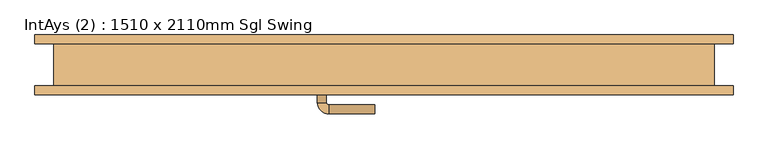
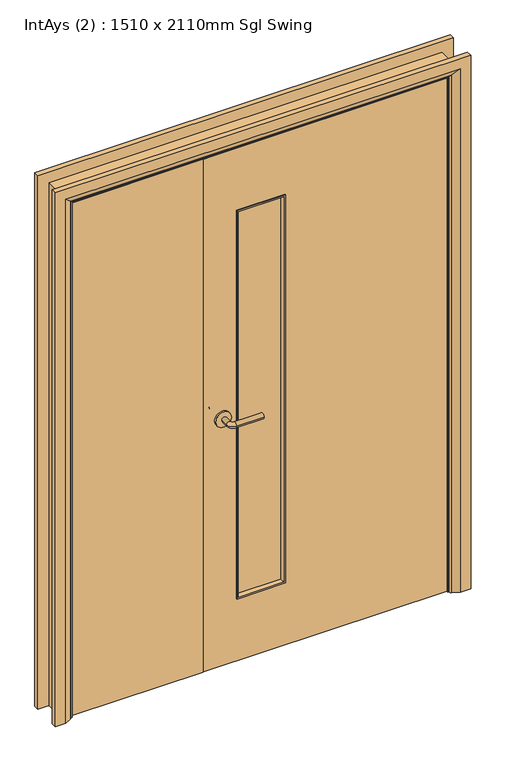
"""IFC4 building model written with IfcOpenShell, lengths in millimetres: door geometry, IntAys (2) : 1510 x 2110mm Sgl Swing."""

import ifcopenshell
import ifcopenshell.guid

model = None  # the IFC model being written
_history = None  # IfcOwnerHistory: only IFC2X3 demands one
_inside = {}  # id of a spatial element -> (the spatial element, [elements in it])
_under = {}  # id of a project, library or spatial element -> (it, [spatial elements below it])
_declared = {}  # id of a project -> (the project, [libraries it declares])
_typed = {}  # id of a type object -> (the type object, [elements of that type])
_made_of = {}  # id of a material, layer set ... -> (it, [elements and type objects made of it])


def new_model(schema):
    """Start an empty IFC model of exactly this schema.

    Asked for "IFC4X3", IfcOpenShell would pick the latest addendum, in which some entities
    have other attributes; the version numbers below select the first issue.
    IFC2X3 requires an IfcOwnerHistory on every rooted entity: one is made here for all.
    """
    global model, _history
    if schema == "IFC4X3":
        model = ifcopenshell.file(schema_version=(4, 3, 0, 0))
    else:
        model = ifcopenshell.file(schema=schema)
    _inside.clear()
    _under.clear()
    _declared.clear()
    _typed.clear()
    _made_of.clear()
    _history = None
    if model.schema == "IFC2X3":
        org = make("IfcOrganization", Name="unknown")
        user = make(
            "IfcPersonAndOrganization",
            ThePerson=make("IfcPerson", FamilyName="unknown"),
            TheOrganization=org,
        )
        app = make(
            "IfcApplication",
            ApplicationDeveloper=org,
            Version="unknown",
            ApplicationFullName="unknown",
            ApplicationIdentifier="unknown",
        )
        _history = make(
            "IfcOwnerHistory",
            OwningUser=user,
            OwningApplication=app,
            ChangeAction="ADDED",
            CreationDate=0,
        )
    return model


def make(cls, **values):
    """One entity of the class cls with the attributes given. An attribute that is None is left unset."""
    return model.create_entity(
        cls, **{name: value for name, value in values.items() if value is not None}
    )


def rooted(cls, **values):
    """An entity with a GlobalId (a new one), such as an element, a storey or a relation."""
    return make(cls, GlobalId=ifcopenshell.guid.new(), OwnerHistory=_history, **values)


def si_unit(unit_type, name, prefix=None):
    """IfcSIUnit, for example si_unit("LENGTHUNIT", "METRE", prefix="MILLI")."""
    return make("IfcSIUnit", UnitType=unit_type, Prefix=prefix, Name=name)


def assignment(units):
    """IfcUnitAssignment: the units of a project."""
    return None if units is None else make("IfcUnitAssignment", Units=units)


def point(xyz):
    """IfcCartesianPoint."""
    return None if xyz is None else make("IfcCartesianPoint", Coordinates=xyz)


def direction(xyz):
    """IfcDirection."""
    return None if xyz is None else make("IfcDirection", DirectionRatios=xyz)


def frame(location, z_axis=None, x_axis=None):
    """IfcAxis2Placement3D, a coordinate frame: its origin and axes. An axis left out is left unset."""
    return make(
        "IfcAxis2Placement3D",
        Location=point(location),
        Axis=direction(z_axis),
        RefDirection=direction(x_axis),
    )


def frame_2d(location, x_axis=None):
    """IfcAxis2Placement2D, a coordinate frame in the plane: its origin and x axis."""
    return make(
        "IfcAxis2Placement2D", Location=point(location), RefDirection=direction(x_axis)
    )


def origin():
    """The frame at (0, 0, 0) with its axes left unset."""
    return frame((0.0, 0.0, 0.0))


def place(relative_to, where):
    """IfcLocalPlacement: puts the frame where relative to a parent placement (None: the world)."""
    return make(
        "IfcLocalPlacement", PlacementRelTo=relative_to, RelativePlacement=where
    )


def context(
    kind, dimensions, precision=None, world=None, true_north=None, identifier=None
):
    """IfcGeometricRepresentationContext, for example the 3D "Model" context."""
    return make(
        "IfcGeometricRepresentationContext",
        ContextIdentifier=identifier,
        ContextType=kind,
        CoordinateSpaceDimension=dimensions,
        Precision=precision,
        WorldCoordinateSystem=world,
        TrueNorth=true_north,
    )


def project(units=None, contexts=None):
    """IfcProject with its units and contexts."""
    return rooted(
        "IfcProject",
        Name="project",
        RepresentationContexts=contexts,
        UnitsInContext=assignment(units),
    )


def spatial(cls, under=None, at=None, **own):
    """A site, building, storey or space (cls), placed at a placement, below another one or the project."""
    s = rooted(cls, ObjectPlacement=at, **own)
    if under is not None:
        _under.setdefault(under.id(), (under, []))[1].append(s)
    return s


def polyline(points):
    """IfcPolyline through the points."""
    return make("IfcPolyline", Points=[point(p) for p in points])


def circle_curve(where, radius):
    """IfcCircle in the frame where."""
    return make("IfcCircle", Position=where, Radius=radius)


def ellipse_curve(where, semi_axis1, semi_axis2):
    """IfcEllipse in the frame where."""
    return make(
        "IfcEllipse", Position=where, SemiAxis1=semi_axis1, SemiAxis2=semi_axis2
    )


def trimmed(basis, trim1, trim2, sense, master):
    """IfcTrimmedCurve: the piece of a basis curve between two trims."""
    return make(
        "IfcTrimmedCurve",
        BasisCurve=basis,
        Trim1=trim1,
        Trim2=trim2,
        SenseAgreement=sense,
        MasterRepresentation=master,
    )


def segment(curve, same_sense, transition):
    """IfcCompositeCurveSegment."""
    return make(
        "IfcCompositeCurveSegment",
        Transition=transition,
        SameSense=same_sense,
        ParentCurve=curve,
    )


def composite_curve(segments, self_intersect=None):
    """IfcCompositeCurve: segments joined end to end."""
    return make("IfcCompositeCurve", Segments=segments, SelfIntersect=self_intersect)


def outline(outer, holes=None, kind="AREA"):
    """IfcArbitraryClosedProfileDef: a profile drawn as a closed curve; with holes, ...WithVoids."""
    if holes is None:
        return make("IfcArbitraryClosedProfileDef", ProfileType=kind, OuterCurve=outer)
    return make(
        "IfcArbitraryProfileDefWithVoids",
        ProfileType=kind,
        OuterCurve=outer,
        InnerCurves=holes,
    )


def extrude(swept, where, along, depth):
    """IfcExtrudedAreaSolid: the profile swept, set in the frame where, extruded along a direction by depth."""
    return make(
        "IfcExtrudedAreaSolid",
        SweptArea=swept,
        Position=where,
        ExtrudedDirection=direction(along),
        Depth=depth,
    )


def faces_of(points, faces, orient=None, outer=None):
    """IfcFace entities. A face is a list of loops; a loop is a list of indices into points, from 0.

    orient and outer hold one flag for each loop. By default every Orientation is true, the
    first loop of a face is its IfcFaceOuterBound and the others are IfcFaceBound.
    """
    made = []
    for i, loops in enumerate(faces):
        bounds = []
        for j, loop in enumerate(loops):
            is_outer = j == 0 if outer is None else outer[i][j]
            bounds.append(
                make(
                    "IfcFaceOuterBound" if is_outer else "IfcFaceBound",
                    Bound=make("IfcPolyLoop", Polygon=[points[k] for k in loop]),
                    Orientation=True if orient is None else orient[i][j],
                )
            )
        made.append(make("IfcFace", Bounds=bounds))
    return made


def faceted_brep(points, faces, orient=None, outer=None, voids=None):
    """IfcFacetedBrep: a solid bounded by flat faces; with voids (closed shells), ...WithVoids."""
    shared = [point(p) for p in points]
    hull = make("IfcClosedShell", CfsFaces=faces_of(shared, faces, orient, outer))
    if voids is None:
        return make("IfcFacetedBrep", Outer=hull)
    return make(
        "IfcFacetedBrepWithVoids",
        Outer=hull,
        Voids=[
            make(cls, CfsFaces=faces_of(shared, fs, o, b)) for cls, fs, o, b in voids
        ],
    )


def shape(context_of_items, identifier, shape_type, items):
    """IfcShapeRepresentation: the items that make up one representation, for example the "Body"."""
    return make(
        "IfcShapeRepresentation",
        ContextOfItems=context_of_items,
        RepresentationIdentifier=identifier,
        RepresentationType=shape_type,
        Items=items,
    )


def source(mapping_origin, context_of_items, identifier, shape_type, items):
    """IfcRepresentationMap: a shape defined once, which mapped items show again and again."""
    return make(
        "IfcRepresentationMap",
        MappingOrigin=mapping_origin,
        MappedRepresentation=shape(context_of_items, identifier, shape_type, items),
    )


def transform(
    local_origin,
    x_axis=None,
    y_axis=None,
    z_axis=None,
    scale=None,
    scale2=None,
    scale3=None,
    uniform=True,
):
    """IfcCartesianTransformationOperator3D, or its non-uniform kind. x_axis, y_axis, z_axis: its Axis1, 2, 3."""
    if uniform:
        return make(
            "IfcCartesianTransformationOperator3D",
            Axis1=direction(x_axis),
            Axis2=direction(y_axis),
            LocalOrigin=point(local_origin),
            Scale=scale,
            Axis3=direction(z_axis),
        )
    return make(
        "IfcCartesianTransformationOperator3DnonUniform",
        Axis1=direction(x_axis),
        Axis2=direction(y_axis),
        LocalOrigin=point(local_origin),
        Scale=scale,
        Axis3=direction(z_axis),
        Scale2=scale2,
        Scale3=scale3,
    )


def mapped(mapping_source, mapping_target):
    """IfcMappedItem: shows the shape of a source again, moved by a transform."""
    return make(
        "IfcMappedItem", MappingSource=mapping_source, MappingTarget=mapping_target
    )


def made_of(thing, what):
    """Note that an element or type object is made of a material, layer set ...; save() writes the relation."""
    if what is not None:
        _made_of.setdefault(what.id(), (what, []))[1].append(thing)
    return thing


def element(
    cls,
    number,
    at=None,
    inside=None,
    cuts=None,
    type_object=None,
    material=None,
    context=None,
    identifier="Body",
    shape_type=None,
    held_by="IfcProductDefinitionShape",
    body=None,
    shapes=None,
    **own,
):
    """One element of the class cls, such as IfcWall. Its Tag is "e" and its number.

    at: its placement. inside: the storey or other place that contains it. cuts: it is an
    opening in that element (IfcRelVoidsElement). A single representation is given by context,
    identifier, shape_type and body (its items); several are given by shapes. held_by: the class
    of the entity that holds the representations. save() writes the other relations.
    """
    e = rooted(cls, Tag="e%d" % number, ObjectPlacement=at, **own)
    if body is not None:
        shapes = [shape(context, identifier, shape_type, body)]
    if shapes is not None:
        e.Representation = make(held_by, Representations=shapes)
    if inside is not None:
        _inside.setdefault(inside.id(), (inside, []))[1].append(e)
    if cuts is not None:
        rooted(
            "IfcRelVoidsElement", RelatingBuildingElement=cuts, RelatedOpeningElement=e
        )
    if type_object is not None:
        _typed.setdefault(type_object.id(), (type_object, []))[1].append(e)
    return made_of(e, material)


def aggregate(whole, parts):
    """IfcRelAggregates: a whole, such as a stair, and the parts it consists of."""
    return rooted("IfcRelAggregates", RelatingObject=whole, RelatedObjects=parts)


def save(model, path):
    """Write the relations noted so far, then the file.

    IfcRelAggregates (storeys below a building ...), IfcRelContainedInSpatialStructure (elements
    in a storey), IfcRelDefinesByType, IfcRelAssociatesMaterial and IfcRelDeclares: one each for
    every whole, place, type object, material and project.
    """
    for whole, parts in _under.values():
        aggregate(whole, parts)
    for where, things in _inside.values():
        rooted(
            "IfcRelContainedInSpatialStructure",
            RelatedElements=things,
            RelatingStructure=where,
        )
    for kind, things in _typed.values():
        rooted("IfcRelDefinesByType", RelatedObjects=things, RelatingType=kind)
    for what, things in _made_of.values():
        rooted("IfcRelAssociatesMaterial", RelatedObjects=things, RelatingMaterial=what)
    for by, libraries in _declared.values():
        rooted("IfcRelDeclares", RelatingContext=by, RelatedDefinitions=libraries)
    model.write(path)


def plane_surface(at):
    """IfcPlane: the flat surface through the origin of the frame at, square to its z axis."""
    return make("IfcPlane", Position=at)


def cylinder_surface(at, radius):
    """IfcCylindricalSurface: all points at the distance radius from the z axis of the frame at."""
    return make("IfcCylindricalSurface", Position=at, Radius=radius)


def revolved_surface(curve, axis_point, axis_direction):
    """IfcSurfaceOfRevolution: the curve turned about the line through axis_point along axis_direction."""
    return make(
        "IfcSurfaceOfRevolution",
        SweptCurve=make("IfcArbitraryOpenProfileDef", ProfileType="CURVE", Curve=curve),
        AxisPosition=make("IfcAxis1Placement", Location=point(axis_point), Axis=direction(axis_direction)),
    )


def advanced_brep(points, edges, surfaces, faces):
    """IfcAdvancedBrep: a solid bounded by faces that lie on surfaces and meet in shared edges.

    An edge is (start, end): straight between two places in points (the first is 0);
    or (start, end, curve); or (start, end, curve, False) where it runs against its curve.
    A face is (place in surfaces, loops), or (place, loops, False) where it looks against
    its surface's normal. A loop lists edges by number (the first is 1), with a minus sign
    where the edge is run from its end to its start. The first loop is the outer one.
    """
    corners = [point(p) for p in points]
    vertices = [make("IfcVertexPoint", VertexGeometry=c) for c in corners]
    made = []
    for start, end, *more in edges:
        made.append(
            make(
                "IfcEdgeCurve",
                EdgeStart=vertices[start],
                EdgeEnd=vertices[end],
                EdgeGeometry=more[0] if more else make("IfcPolyline", Points=[corners[start], corners[end]]),
                SameSense=more[1] if len(more) > 1 else True,
            )
        )
    hull = []
    for where, loops, *sense in faces:
        bounds = []
        for j, loop in enumerate(loops):
            ring = [make("IfcOrientedEdge", EdgeElement=made[abs(k) - 1], Orientation=k > 0) for k in loop]
            bounds.append(
                make(
                    "IfcFaceOuterBound" if j == 0 else "IfcFaceBound",
                    Bound=make("IfcEdgeLoop", EdgeList=ring),
                    Orientation=True,
                )
            )
        hull.append(make("IfcAdvancedFace", Bounds=bounds, FaceSurface=surfaces[where], SameSense=sense[0] if sense else True))
    return make("IfcAdvancedBrep", Outer=make("IfcClosedShell", CfsFaces=hull))


def intays_2_1510_x_2110mm_sgl_swing_7badbe2f(model_context):
    return source(origin(), model_context, "Body", "SolidModel", [
        advanced_brep(
        [(88.5, -7.5, 1000.0), (108.5, -7.5, 1000.0), (88.5, 22.5, 1000.0), (108.5, 22.5, 1000.0), (113.5, 27.5, 1000.0), (113.5, 47.5, 1000.0), (218.5, 47.5, 1000.0), (218.5, 27.5, 1000.0)],
        [
            (0, 1, circle_curve(frame((98.5, -7.5, 1000.0), z_axis=(0.0, -1.0, 0.0), x_axis=(1.0, 0.0, 0.0)), 10.0)),
            (1, 0, circle_curve(frame((98.5, -7.5, 1000.0), z_axis=(0.0, -1.0, 0.0), x_axis=(1.0, 0.0, 0.0)), 10.0)),
            (0, 2),
            (2, 3, circle_curve(frame((98.5, 22.5, 1000.0), z_axis=(0.0, -1.0, 0.0), x_axis=(1.0, 0.0, 0.0)), 10.0)),
            (3, 1),
            (3, 2, circle_curve(frame((98.5, 22.5, 1000.0), z_axis=(0.0, -1.0, 0.0), x_axis=(1.0, 0.0, 0.0)), 10.0)),
            (4, 3, circle_curve(frame((113.5, 22.5, 1000.0), z_axis=(0.0, 0.0, 1.0), x_axis=(-1.0, 0.0, 0.0)), 5.0)),
            (2, 5, circle_curve(frame((113.5, 22.5, 1000.0), z_axis=(0.0, 0.0, -1.0), x_axis=(-1.0, 0.0, 0.0)), 25.0)),
            (5, 4, circle_curve(frame((113.5, 37.5, 1000.0), z_axis=(-1.0, 0.0, 0.0), x_axis=(0.0, -1.0, 0.0)), 10.0)),
            (4, 5, circle_curve(frame((113.5, 37.5, 1000.0), z_axis=(-1.0, 0.0, 0.0), x_axis=(0.0, -1.0, 0.0)), 10.0)),
            (6, 7, circle_curve(frame((218.5, 37.5, 1000.0), z_axis=(1.0, 0.0, 0.0), x_axis=(0.0, -1.0, 0.0)), 10.0)),
            (7, 6, circle_curve(frame((218.5, 37.5, 1000.0), z_axis=(1.0, 0.0, 0.0), x_axis=(0.0, -1.0, 0.0)), 10.0)),
            (5, 6),
            (7, 4),
        ],
        [
            plane_surface(frame((98.5, -7.5, 1000.0), z_axis=(0.0, -1.0, 0.0), x_axis=(0.0, 0.0, 1.0))),
            cylinder_surface(frame((98.5, -7.5, 1000.0), z_axis=(0.0, -1.0, 0.0), x_axis=(1.0, 0.0, 0.0)), 10.0),
            revolved_surface(trimmed(ellipse_curve(frame((98.5, 22.5, 1000.0), z_axis=(0.0, -1.0, 0.0), x_axis=(1.0, 0.0, 0.0)), 10.0, 10.0), [point((88.5, 22.5, 1000.0))], [point((108.5, 22.5, 1000.0))], True, "CARTESIAN"), (113.5, 22.5, 1000.0), (0.0, 0.0, -1.0)),
            revolved_surface(trimmed(ellipse_curve(frame((98.5, 22.5, 1000.0), z_axis=(0.0, -1.0, 0.0), x_axis=(1.0, 0.0, 0.0)), 10.0, 10.0), [point((108.5, 22.5, 1000.0))], [point((88.5, 22.5, 1000.0))], True, "CARTESIAN"), (113.5, 22.5, 1000.0), (0.0, 0.0, -1.0)),
            plane_surface(frame((218.5, 37.5, 1000.0), z_axis=(1.0, 0.0, 0.0), x_axis=(0.0, 0.0, 1.0))),
            cylinder_surface(frame((113.5, 37.5, 1000.0), z_axis=(-1.0, 0.0, 0.0), x_axis=(0.0, -1.0, 0.0)), 10.0),
        ],
        [
            (0, [[1, 2]]),
            (1, [[-1, 3, 4, 5]]),
            (1, [[-2, -5, 6, -3]]),
            (2, [[7, -4, 8, 9]]),
            (3, [[-8, -6, -7, 10]]),
            (4, [[11, 12]]),
            (5, [[-9, 13, -12, 14]]),
            (5, [[-10, -14, -11, -13]]),
        ],
    ),
        extrude(outline(composite_curve([segment(trimmed(circle_curve(frame_2d((1000.0, 96.0)), 30.0), [point((1000.0, 66.0))], [point((1000.0, 126.0))], False, "CARTESIAN"), True, "CONTINUOUS"), segment(trimmed(circle_curve(frame_2d((1000.0, 96.0)), 30.0), [point((1000.0, 126.0))], [point((1000.0, 66.0))], False, "CARTESIAN"), True, "CONTINUOUS")], self_intersect=False)), frame((0.0, -15.5, 0.0), z_axis=(0.0, 1.0, 0.0), x_axis=(0.0, 0.0, 1.0)), (0.0, 0.0, 1.0), 8.0),
        advanced_brep(
        [(88.5, -55.5, 1000.0), (108.5, -55.5, 1000.0), (108.5, -85.5, 1000.0), (88.5, -85.5, 1000.0), (113.5, -90.5, 1000.0), (113.5, -110.5, 1000.0), (218.5, -110.5, 1000.0), (218.5, -90.5, 1000.0)],
        [
            (0, 1, circle_curve(frame((98.5, -55.5, 1000.0), z_axis=(0.0, 1.0, 0.0), x_axis=(1.0, 0.0, 0.0)), 10.0)),
            (1, 0, circle_curve(frame((98.5, -55.5, 1000.0), z_axis=(0.0, 1.0, 0.0), x_axis=(1.0, 0.0, 0.0)), 10.0)),
            (1, 2),
            (2, 3, circle_curve(frame((98.5, -85.5, 1000.0), z_axis=(0.0, 1.0, 0.0), x_axis=(1.0, 0.0, 0.0)), 10.0)),
            (3, 0),
            (3, 2, circle_curve(frame((98.5, -85.5, 1000.0), z_axis=(0.0, 1.0, 0.0), x_axis=(1.0, 0.0, 0.0)), 10.0)),
            (4, 5, circle_curve(frame((113.5, -100.5, 1000.0), z_axis=(-1.0, 0.0, 0.0), x_axis=(0.0, 1.0, 0.0)), 10.0)),
            (5, 3, circle_curve(frame((113.5, -85.5, 1000.0), z_axis=(0.0, 0.0, -1.0), x_axis=(-1.0, 0.0, 0.0)), 25.0)),
            (2, 4, circle_curve(frame((113.5, -85.5, 1000.0), z_axis=(0.0, 0.0, 1.0), x_axis=(-1.0, 0.0, 0.0)), 5.0)),
            (5, 4, circle_curve(frame((113.5, -100.5, 1000.0), z_axis=(-1.0, 0.0, 0.0), x_axis=(0.0, 1.0, 0.0)), 10.0)),
            (6, 7, circle_curve(frame((218.5, -100.5, 1000.0), z_axis=(1.0, 0.0, 0.0), x_axis=(0.0, 1.0, 0.0)), 10.0)),
            (7, 6, circle_curve(frame((218.5, -100.5, 1000.0), z_axis=(1.0, 0.0, 0.0), x_axis=(0.0, 1.0, 0.0)), 10.0)),
            (4, 7),
            (6, 5),
        ],
        [
            plane_surface(frame((98.5, -55.5, 1000.0), z_axis=(0.0, 1.0, 0.0), x_axis=(0.0, 0.0, 1.0))),
            cylinder_surface(frame((98.5, -55.5, 1000.0), z_axis=(0.0, 1.0, 0.0), x_axis=(1.0, 0.0, 0.0)), 10.0),
            revolved_surface(trimmed(ellipse_curve(frame((98.5, -85.5, 1000.0), z_axis=(0.0, -1.0, 0.0), x_axis=(1.0, 0.0, 0.0)), 10.0, 10.0), [point((88.5, -85.5, 1000.0))], [point((108.5, -85.5, 1000.0))], True, "CARTESIAN"), (113.5, -85.5, 1000.0), (0.0, 0.0, -1.0)),
            revolved_surface(trimmed(ellipse_curve(frame((98.5, -85.5, 1000.0), z_axis=(0.0, -1.0, 0.0), x_axis=(1.0, 0.0, 0.0)), 10.0, 10.0), [point((108.5, -85.5, 1000.0))], [point((88.5, -85.5, 1000.0))], True, "CARTESIAN"), (113.5, -85.5, 1000.0), (0.0, 0.0, -1.0)),
            plane_surface(frame((218.5, -100.5, 1000.0), z_axis=(1.0, 0.0, 0.0), x_axis=(0.0, 0.0, 1.0))),
            cylinder_surface(frame((113.5, -100.5, 1000.0), z_axis=(-1.0, 0.0, 0.0), x_axis=(0.0, 1.0, 0.0)), 10.0),
        ],
        [
            (0, [[1, 2]]),
            (1, [[3, 4, 5, -2]]),
            (1, [[-5, 6, -3, -1]]),
            (2, [[7, 8, -4, 9]]),
            (3, [[10, -9, -6, -8]]),
            (4, [[11, 12]]),
            (5, [[13, -11, 14, -7]]),
            (5, [[-14, -12, -13, -10]]),
        ],
    ),
        extrude(outline(composite_curve([segment(trimmed(circle_curve(frame_2d((1000.0, 96.0)), 30.0), [point((1000.0, 66.0))], [point((1000.0, 126.0))], False, "CARTESIAN"), True, "CONTINUOUS"), segment(trimmed(circle_curve(frame_2d((1000.0, 96.0)), 30.0), [point((1000.0, 126.0))], [point((1000.0, 66.0))], False, "CARTESIAN"), True, "CONTINUOUS")], self_intersect=False)), frame((0.0, -55.5, 0.0), z_axis=(0.0, 1.0, 0.0), x_axis=(0.0, 0.0, 1.0)), (0.0, 0.0, 1.0), 8.0),
        extrude(outline(polyline([(2102.0, -508.0), (0.0, -508.0), (0.0, -476.0), (2070.0, -476.0), (2070.0, 954.0), (0.0, 954.0), (0.0, 986.0), (2102.0, 986.0), (2102.0, -508.0)])), frame((0.0, -47.5, 0.0), z_axis=(0.0, 1.0, 0.0), x_axis=(0.0, 0.0, 1.0)), (0.0, 0.0, 1.0), 95.0),
        advanced_brep(
        [(-551.0, 67.5, 0.0), (-511.0, 67.5, 0.0), (-485.0, 53.5, 0.0), (-481.0, 47.5, 0.0), (-551.0, 47.5, 0.0), (-551.0, 47.5, 2145.0), (-551.0, 67.5, 2145.0), (-481.0, 47.5, 2075.0), (959.0, 47.5, 2075.0), (959.0, 47.5, 0.0), (1029.0, 47.5, 0.0), (1029.0, 47.5, 2145.0), (-485.0, 53.5, 2079.0), (-511.0, 67.5, 2105.0), (1029.0, 67.5, 2145.0), (1029.0, 67.5, 0.0), (989.0, 67.5, 0.0), (989.0, 67.5, 2105.0), (963.0, 53.5, 0.0), (963.0, 53.5, 2079.0)],
        [
            (0, 1),
            (1, 2),
            (2, 3, circle_curve(frame((-489.0, 46.5, 0.0), z_axis=(0.0, 0.0, -1.0), x_axis=(-1.0, 0.0, 0.0)), 8.0622577)),
            (3, 4),
            (4, 0),
            (4, 5),
            (5, 6),
            (6, 0),
            (3, 7),
            (7, 8),
            (8, 9),
            (9, 10),
            (10, 11),
            (11, 5),
            (2, 12),
            (12, 7, ellipse_curve(frame((-489.0, 46.5, 2083.0), z_axis=(-0.7071067811865475, 0.0, -0.7071067811865475), x_axis=(0.7071067811865474, 0.0, -0.7071067811865476)), 11.4017543, 8.0622577)),
            (1, 13),
            (13, 12),
            (6, 14),
            (14, 15),
            (15, 16),
            (16, 17),
            (17, 13),
            (10, 15),
            (14, 11),
            (9, 18, circle_curve(frame((967.0, 46.5, 0.0), z_axis=(0.0, 0.0, -1.0), x_axis=(1.0, 0.0, 0.0)), 8.0622577)),
            (18, 16),
            (19, 18),
            (8, 19, ellipse_curve(frame((967.0, 46.5, 2083.0), z_axis=(0.7071067811865475, 0.0, -0.7071067811865475), x_axis=(0.7071067811865474, 0.0, 0.7071067811865476)), 11.4017543, 8.0622577)),
            (19, 17),
            (12, 19),
        ],
        [
            plane_surface(frame((-481.0, 47.5, 0.0), z_axis=(0.0, 0.0, -1.0), x_axis=(0.0, 1.0, 0.0))),
            plane_surface(frame((-551.0, 67.5, 0.0), z_axis=(-1.0, 0.0, 0.0), x_axis=(0.0, 0.0, 1.0))),
            plane_surface(frame((-551.0, 47.5, 0.0), z_axis=(0.0, -1.0, 0.0), x_axis=(0.0, 0.0, 1.0))),
            cylinder_surface(frame((-489.0, 46.5, 0.0), z_axis=(0.0, 0.0, -1.0), x_axis=(-1.0, 0.0, 0.0)), 8.0622577),
            plane_surface(frame((-485.0, 53.5, 0.0), z_axis=(0.4740998230350183, 0.8804710999221749, 0.0), x_axis=(0.0, 0.0, 1.0))),
            plane_surface(frame((-511.0, 67.5, 0.0), z_axis=(0.0, 1.0, 0.0), x_axis=(0.0, 0.0, 1.0))),
            plane_surface(frame((1029.0, 67.5, 2145.0), z_axis=(1.0, 0.0, 0.0), x_axis=(0.0, 0.0, -1.0))),
            plane_surface(frame((959.0, 47.5, 0.0), z_axis=(0.0, 0.0, -1.0), x_axis=(0.0, 1.0, 0.0))),
            cylinder_surface(frame((967.0, 46.5, 2075.0), z_axis=(0.0, 0.0, 1.0), x_axis=(1.0, 0.0, 0.0)), 8.0622577),
            plane_surface(frame((963.0, 53.5, 2079.0), z_axis=(-0.4740998230350183, 0.8804710999221749, 0.0), x_axis=(0.0, 0.0, -1.0))),
            plane_surface(frame((-551.0, 67.5, 2145.0), z_axis=(0.0, 0.0, 1.0), x_axis=(1.0, 0.0, 0.0))),
            cylinder_surface(frame((-481.0, 46.5, 2083.0), z_axis=(-1.0, 0.0, 0.0), x_axis=(0.0, 0.0, 1.0)), 8.0622577),
            plane_surface(frame((-485.0, 53.5, 2079.0), z_axis=(0.0, 0.8804710999221749, -0.4740998230350183), x_axis=(1.0, 0.0, 0.0))),
        ],
        [
            (0, [[1, 2, 3, 4, 5]]),
            (1, [[6, 7, 8, -5]]),
            (2, [[9, 10, 11, 12, 13, 14, -6, -4]]),
            (3, [[15, 16, -9, -3]]),
            (4, [[17, 18, -15, -2]]),
            (5, [[-8, 19, 20, 21, 22, 23, -17, -1]]),
            (6, [[-13, 24, -20, 25]]),
            (7, [[-24, -12, 26, 27, -21]]),
            (8, [[28, -26, -11, 29]]),
            (9, [[-22, -27, -28, 30]]),
            (10, [[-14, -25, -19, -7]]),
            (11, [[31, -29, -10, -16]]),
            (12, [[-23, -30, -31, -18]]),
        ],
    ),
        advanced_brep(
        [(1029.0, -67.5, 0.0), (989.0, -67.5, 0.0), (963.0, -53.5, 0.0), (959.0, -47.5, 0.0), (1029.0, -47.5, 0.0), (1029.0, -47.5, 2145.0), (1029.0, -67.5, 2145.0), (959.0, -47.5, 2075.0), (-481.0, -47.5, 2075.0), (-481.0, -47.5, 0.0), (-551.0, -47.5, 0.0), (-551.0, -47.5, 2145.0), (963.0, -53.5, 2079.0), (989.0, -67.5, 2105.0), (-551.0, -67.5, 2145.0), (-551.0, -67.5, 0.0), (-511.0, -67.5, 0.0), (-511.0, -67.5, 2105.0), (-485.0, -53.5, 0.0), (-485.0, -53.5, 2079.0)],
        [
            (0, 1),
            (1, 2),
            (2, 3, circle_curve(frame((967.0, -46.5, 0.0), z_axis=(0.0, 0.0, -1.0), x_axis=(1.0, 0.0, 0.0)), 8.0622577)),
            (3, 4),
            (4, 0),
            (4, 5),
            (5, 6),
            (6, 0),
            (3, 7),
            (7, 8),
            (8, 9),
            (9, 10),
            (10, 11),
            (11, 5),
            (2, 12),
            (12, 7, ellipse_curve(frame((967.0, -46.5, 2083.0), z_axis=(0.7071067811865475, 0.0, -0.7071067811865475), x_axis=(-0.7071067811865474, 0.0, -0.7071067811865476)), 11.4017543, 8.0622577)),
            (1, 13),
            (13, 12),
            (6, 14),
            (14, 15),
            (15, 16),
            (16, 17),
            (17, 13),
            (10, 15),
            (14, 11),
            (9, 18, circle_curve(frame((-489.0, -46.5, 0.0), z_axis=(0.0, 0.0, -1.0), x_axis=(-1.0, 0.0, 0.0)), 8.0622577)),
            (18, 16),
            (19, 18),
            (8, 19, ellipse_curve(frame((-489.0, -46.5, 2083.0), z_axis=(-0.7071067811865475, 0.0, -0.7071067811865475), x_axis=(-0.7071067811865474, 0.0, 0.7071067811865476)), 11.4017543, 8.0622577)),
            (19, 17),
            (12, 19),
        ],
        [
            plane_surface(frame((959.0, -47.5, 0.0), z_axis=(0.0, 0.0, -1.0), x_axis=(0.0, 1.0, 0.0))),
            plane_surface(frame((1029.0, -67.5, 0.0), z_axis=(1.0, 0.0, 0.0), x_axis=(0.0, 0.0, 1.0))),
            plane_surface(frame((1029.0, -47.5, 0.0), z_axis=(0.0, 1.0, 0.0), x_axis=(0.0, 0.0, 1.0))),
            cylinder_surface(frame((967.0, -46.5, 0.0), z_axis=(0.0, 0.0, -1.0), x_axis=(1.0, 0.0, 0.0)), 8.0622577),
            plane_surface(frame((963.0, -53.5, 0.0), z_axis=(-0.4740998230350126, -0.8804710999221779, 0.0), x_axis=(0.0, 0.0, 1.0))),
            plane_surface(frame((989.0, -67.5, 0.0), z_axis=(0.0, -1.0, 0.0), x_axis=(0.0, 0.0, 1.0))),
            plane_surface(frame((-551.0, -67.5, 2145.0), z_axis=(-1.0, 0.0, 0.0), x_axis=(0.0, 0.0, -1.0))),
            plane_surface(frame((-481.0, -47.5, 0.0), z_axis=(0.0, 0.0, -1.0), x_axis=(0.0, 1.0, 0.0))),
            cylinder_surface(frame((-489.0, -46.5, 2075.0), z_axis=(0.0, 0.0, 1.0), x_axis=(-1.0, 0.0, 0.0)), 8.0622577),
            plane_surface(frame((-485.0, -53.5, 2079.0), z_axis=(0.4740998230350183, -0.8804710999221749, 0.0), x_axis=(0.0, 0.0, -1.0))),
            plane_surface(frame((1029.0, -67.5, 2145.0), z_axis=(0.0, 0.0, 1.0), x_axis=(-1.0, 0.0, 0.0))),
            cylinder_surface(frame((959.0, -46.5, 2083.0), z_axis=(1.0, 0.0, 0.0), x_axis=(0.0, 0.0, 1.0)), 8.0622577),
            plane_surface(frame((963.0, -53.5, 2079.0), z_axis=(0.0, -0.8804710999221763, -0.4740998230350154), x_axis=(-1.0, 0.0, 0.0))),
        ],
        [
            (0, [[1, 2, 3, 4, 5]]),
            (1, [[6, 7, 8, -5]]),
            (2, [[9, 10, 11, 12, 13, 14, -6, -4]]),
            (3, [[15, 16, -9, -3]]),
            (4, [[17, 18, -15, -2]]),
            (5, [[-8, 19, 20, 21, 22, 23, -17, -1]]),
            (6, [[-13, 24, -20, 25]]),
            (7, [[-24, -12, 26, 27, -21]]),
            (8, [[28, -26, -11, 29]]),
            (9, [[-22, -27, -28, 30]]),
            (10, [[-14, -25, -19, -7]]),
            (11, [[31, -29, -10, -16]]),
            (12, [[-23, -30, -31, -18]]),
        ],
    ),
        faceted_brep([(-457.0, -12.5, 0.0), (-476.0, -12.5, 0.0), (-476.0, 19.5, 0.0), (-457.0, 19.5, 0.0), (-457.0, 19.5, 2051.0), (-457.0, -12.5, 2051.0), (-476.0, 19.5, 2070.0), (-476.0, -12.5, 2070.0), (935.0, -12.5, 0.0), (935.0, 19.5, 0.0), (954.0, 19.5, 0.0), (954.0, -12.5, 0.0), (935.0, -12.5, 2051.0), (954.0, -12.5, 2070.0), (954.0, 19.5, 2070.0), (935.0, 19.5, 2051.0)], [[[0, 1, 2, 3]], [[3, 4, 5, 0]], [[2, 6, 4, 3]], [[1, 7, 6, 2]], [[0, 5, 7, 1]], [[8, 9, 10, 11]], [[12, 8, 11, 13]], [[13, 11, 10, 14]], [[14, 10, 9, 15]], [[15, 9, 8, 12]], [[4, 15, 12, 5]], [[6, 14, 15, 4]], [[7, 13, 14, 6]], [[5, 12, 13, 7]]]),
        extrude(outline(polyline([(335.0, -25.5), (335.0, -37.5), (150.0, -37.5), (150.0, -25.5), (335.0, -25.5)])), frame((0.0, 0.0, 257.0), z_axis=(0.0, 0.0, 1.0), x_axis=(1.0, 0.0, 0.0)), (0.0, 0.0, 1.0), 1560.0),
        extrude(outline(polyline([(22.0, -15.5), (22.0, -47.5), (-473.0, -47.5), (-473.0, -15.5), (22.0, -15.5)])), frame((0.0, 0.0, 5.753223), z_axis=(0.0, 0.0, 1.0), x_axis=(1.0, 0.0, 0.0)), (0.0, 0.0, 1.0), 2061.246777),
        extrude(outline(polyline([(5.753223, 951.0), (2067.0, 951.0), (2067.0, 25.0), (5.753223, 25.0), (5.753223, 951.0)]), holes=[polyline([(1817.0, 150.0), (1817.0, 335.0), (257.0, 335.0), (257.0, 150.0), (1817.0, 150.0)])]), frame((0.0, -47.5, 0.0), z_axis=(0.0, 1.0, 0.0), x_axis=(0.0, 0.0, 1.0)), (0.0, 0.0, 1.0), 32.0),
        faceted_brep([(335.0, -12.5, 257.0), (335.0, -12.5, 1817.0), (335.0, -25.5, 1817.0), (335.0, -25.5, 257.0), (323.0, -25.5, 269.0), (323.0, -25.5, 1805.0), (329.0, -12.5, 1811.0), (329.0, -12.5, 263.0), (150.0, -12.5, 1817.0), (150.0, -25.5, 1817.0), (162.0, -25.5, 1805.0), (156.0, -12.5, 1811.0), (150.0, -12.5, 257.0), (150.0, -25.5, 257.0), (162.0, -25.5, 269.0), (156.0, -12.5, 263.0)], [[[0, 1, 2, 3]], [[4, 5, 6, 7]], [[1, 8, 9, 2]], [[5, 10, 11, 6]], [[8, 12, 13, 9]], [[10, 14, 15, 11]], [[3, 2, 9, 13], [5, 4, 14, 10]], [[12, 0, 3, 13]], [[1, 0, 12, 8], [7, 6, 11, 15]], [[14, 4, 7, 15]]]),
        faceted_brep([(150.0, -50.5, 257.0), (150.0, -50.5, 1817.0), (150.0, -37.5, 1817.0), (150.0, -37.5, 257.0), (162.0, -37.5, 269.0), (162.0, -37.5, 1805.0), (156.0, -50.5, 1811.0), (156.0, -50.5, 263.0), (335.0, -50.5, 1817.0), (335.0, -37.5, 1817.0), (323.0, -37.5, 1805.0), (329.0, -50.5, 1811.0), (335.0, -50.5, 257.0), (335.0, -37.5, 257.0), (323.0, -37.5, 269.0), (329.0, -50.5, 263.0)], [[[0, 1, 2, 3]], [[4, 5, 6, 7]], [[1, 8, 9, 2]], [[5, 10, 11, 6]], [[8, 12, 13, 9]], [[10, 14, 15, 11]], [[3, 2, 9, 13], [5, 4, 14, 10]], [[12, 0, 3, 13]], [[1, 0, 12, 8], [7, 6, 11, 15]], [[14, 4, 7, 15]]]),
    ])


if __name__ == "__main__":
    model = new_model("IFC4")
    model_context = context("Model", 3, world=origin())
    ifc_project = project(units=[si_unit("LENGTHUNIT", "METRE", prefix="MILLI")], contexts=[model_context])
    site = spatial("IfcSite", under=ifc_project)
    building = spatial("IfcBuilding", under=site)
    placement = place(None, origin())
    intays_2_1510_x_2110mm_sgl_swing_shape = intays_2_1510_x_2110mm_sgl_swing_7badbe2f(model_context)
    element("IfcDoor", 1, ObjectType="IntAys (2) : 1510 x 2110mm Sgl Swing", at=placement, inside=building, context=model_context, shape_type="MappedRepresentation", body=[
        mapped(intays_2_1510_x_2110mm_sgl_swing_shape, transform((0.0, 0.0, 0.0), x_axis=(1.0, 0.0, 0.0), y_axis=(0.0, 1.0, 0.0), z_axis=(0.0, 0.0, 1.0))),
    ])
    save(model, "model.ifc")

# Revit data of these elements
# Project information
#   Project Status = "Project Status"
#   Client Name = "Revit Project"
#   Project Address = "LIMERICK INSTITUTE of TECHNOLOGY"
#   Project Name = "Commercial Units"
#   Project Number = "01"
# Type "IntAys (2) : 1510 x 2110mm Sgl Swing"
#   Type Mark = "46"
#   Type Comments = "Internal Asymmetric"
#   Operation = "DoubleDoorSingleSwing"
#   Construction Type Id = "SGL"
#   Keynote = "L20"
#   Description = "Internal Asymmetric Door"
#   Analytic Construction = "Large single-glazed windows"
#   Visual Light Transmittance = 0.9
#   VisionPanel Width = 185 mm
#   Thickness = 32 mm
#   Stop Thickness = 19 mm
#   Stop Depth = 32 mm
#   Stile Top Rail = 250 mm
#   Stile Shutting = 125 mm
#   Stile Bottom Rail = 250 mm
#   Solar Heat Gain Coefficient = 0.86
#   Secondary Panel Width = 495 mm
#   Rough Width = 1510 mm
#   Rough Height = 2110 mm
#   Main Panel Width = 926 mm
#   Heat Transfer Coefficient (U) = 5.5617 W/(m²·K)
#   Handle Z Distance = 1000 mm
#   Handle X Distance = 75 mm
#   Handle Length = 350 mm
#   Frame Thickness = 32 mm
#   Door Panel Width = 926 mm
#   Door Panel Thickness = 32 mm
#   Height = 2110 mm
#   Door Panel Offset = 0 mm
#   Structural Tolerance = 8 mm
#   Tolerance = 3 mm
#   UnderCut = 7 mm
#   Width = 1510 mm
#   Door Panel Height = 2060 mm
#   Architrave Setback = 5 mm
#   Vis - Swing Single = yes
#   Vis - Swing Opposing = no
#   Vis - Swing Double = no
#   Vis - Stops = yes
#   Vis - Ironmongery = yes
#   Material Ironmongery = Door - Handle
#   Material Glass = Door - Glazing
#   Material Frame = Door - Frame/Mullion
#   Material Door = Door - Panel
#   Material Beading = Door - Panel
#   Material Architrave = Door - Architrave
#   Handle Style = element 261135
#   Function = (empty or 0)
#   Wall Closure = (empty or 0)
# Element 1 (IfcDoor, "IntAys (2) : 1510 x 2110mm Sgl Swing")
#   Materials on its faces: "Door - Panel", "Door - Architrave", "Door - Handle", "Door - Frame/Mullion", "Door - Glazing"
# Materials
#   "Door - Handle": class "Miscellaneous", colour RGB 0 0 0, transparency 0, Keynote = "P21"
#   "Door - Glazing": class "Miscellaneous", colour RGB 0 0 255, transparency 0.75
#   "Door - Frame/Mullion": class "Wood", colour RGB 212 179 113, transparency 0, Keynote = "L20"
#   "Door - Panel": class "Wood", colour RGB 210 159 95, transparency 0, Keynote = "L20"
#   "Door - Architrave": class "Wood", colour RGB 154 90 5, transparency 0, Keynote = "P20"
